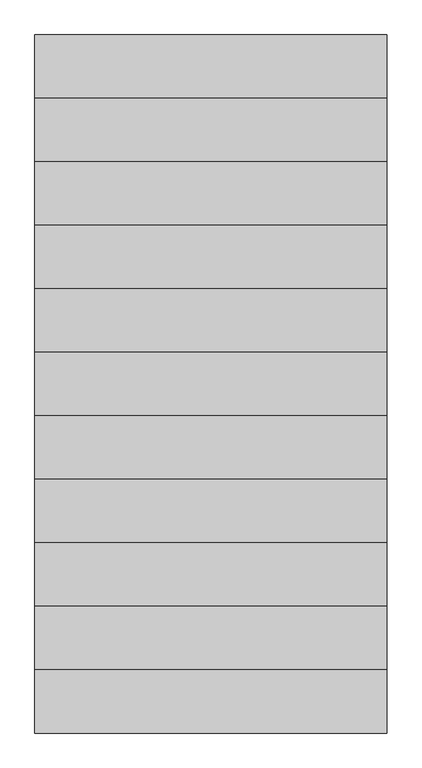
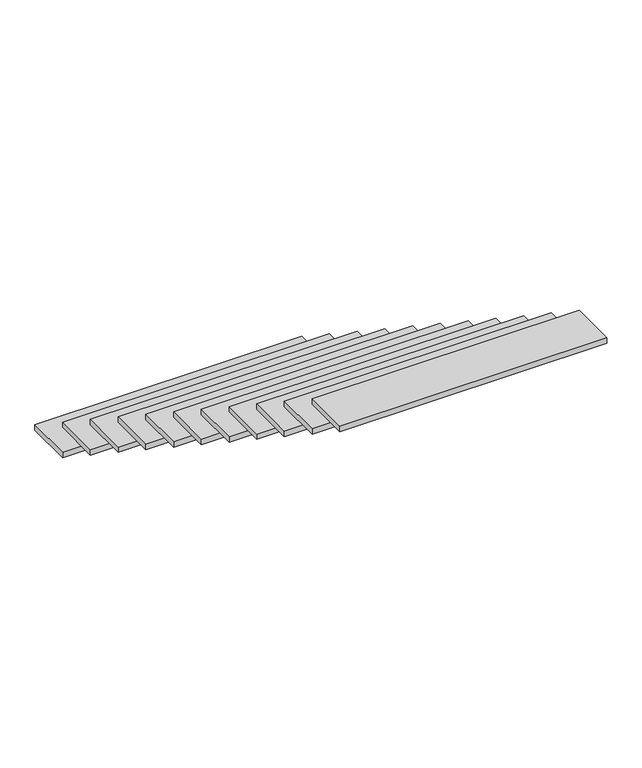
"""IFC4 building model written with IfcOpenShell, lengths in millimetres: stair flight geometry."""

from ifc_helpers import new_model, si_unit, frame, origin, place, context, project, spatial, polyline, outline, extrude, source, transform, mapped, element, save


def stair_flight_fe710d0a(model_context):
    return source(origin(), model_context, "Body", "SweptSolid", [
        extrude(outline(polyline([(16085.3403387, 4647.6066446), (14585.3403387, 4647.6066446), (14585.3403387, 4917.6066446), (16085.3403387, 4917.6066446), (16085.3403387, 4647.6066446)])), frame((0.0, 0.0, 6058.1098901), z_axis=(0.0, 0.0, 1.0), x_axis=(1.0, 0.0, 0.0)), (0.0, 0.0, 1.0), 32.0),
        extrude(outline(polyline([(16085.3403387, 4377.6066446), (14585.3403387, 4377.6066446), (14585.3403387, 4647.6066446), (16085.3403387, 4647.6066446), (16085.3403387, 4377.6066446)])), frame((0.0, 0.0, 6237.2307692), z_axis=(0.0, 0.0, 1.0), x_axis=(1.0, 0.0, 0.0)), (0.0, 0.0, 1.0), 32.0),
        extrude(outline(polyline([(16085.3403387, 4107.6066446), (14585.3403387, 4107.6066446), (14585.3403387, 4377.6066446), (16085.3403387, 4377.6066446), (16085.3403387, 4107.6066446)])), frame((0.0, 0.0, 6416.3516484), z_axis=(0.0, 0.0, 1.0), x_axis=(1.0, 0.0, 0.0)), (0.0, 0.0, 1.0), 32.0),
        extrude(outline(polyline([(16085.3403387, 3837.6066446), (14585.3403387, 3837.6066446), (14585.3403387, 4107.6066446), (16085.3403387, 4107.6066446), (16085.3403387, 3837.6066446)])), frame((0.0, 0.0, 6595.4725275), z_axis=(0.0, 0.0, 1.0), x_axis=(1.0, 0.0, 0.0)), (0.0, 0.0, 1.0), 32.0),
        extrude(outline(polyline([(16085.3403387, 3567.6066446), (14585.3403387, 3567.6066446), (14585.3403387, 3837.6066446), (16085.3403387, 3837.6066446), (16085.3403387, 3567.6066446)])), frame((0.0, 0.0, 6774.5934066), z_axis=(0.0, 0.0, 1.0), x_axis=(1.0, 0.0, 0.0)), (0.0, 0.0, 1.0), 32.0),
        extrude(outline(polyline([(16085.3403387, 3297.6066446), (14585.3403387, 3297.6066446), (14585.3403387, 3567.6066446), (16085.3403387, 3567.6066446), (16085.3403387, 3297.6066446)])), frame((0.0, 0.0, 6953.7142857), z_axis=(0.0, 0.0, 1.0), x_axis=(1.0, 0.0, 0.0)), (0.0, 0.0, 1.0), 32.0),
        extrude(outline(polyline([(16085.3403387, 3027.6066446), (14585.3403387, 3027.6066446), (14585.3403387, 3297.6066446), (16085.3403387, 3297.6066446), (16085.3403387, 3027.6066446)])), frame((0.0, 0.0, 7132.8351648), z_axis=(0.0, 0.0, 1.0), x_axis=(1.0, 0.0, 0.0)), (0.0, 0.0, 1.0), 32.0),
        extrude(outline(polyline([(16085.3403387, 2757.6066446), (14585.3403387, 2757.6066446), (14585.3403387, 3027.6066446), (16085.3403387, 3027.6066446), (16085.3403387, 2757.6066446)])), frame((0.0, 0.0, 7311.956044), z_axis=(0.0, 0.0, 1.0), x_axis=(1.0, 0.0, 0.0)), (0.0, 0.0, 1.0), 32.0),
        extrude(outline(polyline([(16085.3403387, 2487.6066446), (14585.3403387, 2487.6066446), (14585.3403387, 2757.6066446), (16085.3403387, 2757.6066446), (16085.3403387, 2487.6066446)])), frame((0.0, 0.0, 7491.0769231), z_axis=(0.0, 0.0, 1.0), x_axis=(1.0, 0.0, 0.0)), (0.0, 0.0, 1.0), 32.0),
        extrude(outline(polyline([(16085.3403387, 2217.6066446), (14585.3403387, 2217.6066446), (14585.3403387, 2487.6066446), (16085.3403387, 2487.6066446), (16085.3403387, 2217.6066446)])), frame((0.0, 0.0, 7670.1978022), z_axis=(0.0, 0.0, 1.0), x_axis=(1.0, 0.0, 0.0)), (0.0, 0.0, 1.0), 32.0),
        extrude(outline(polyline([(16085.3403387, 1947.6066446), (14585.3403387, 1947.6066446), (14585.3403387, 2217.6066446), (16085.3403387, 2217.6066446), (16085.3403387, 1947.6066446)])), frame((0.0, 0.0, 7849.3186813), z_axis=(0.0, 0.0, 1.0), x_axis=(1.0, 0.0, 0.0)), (0.0, 0.0, 1.0), 32.0),
    ])


if __name__ == "__main__":
    model = new_model("IFC4")
    model_context = context("Model", 3, world=origin())
    ifc_project = project(units=[si_unit("LENGTHUNIT", "METRE", prefix="MILLI")], contexts=[model_context])
    site = spatial("IfcSite", under=ifc_project)
    building = spatial("IfcBuilding", under=site)
    placement = place(None, origin())
    stair_flight_shape = stair_flight_fe710d0a(model_context)
    element("IfcStairFlight", 1, at=placement, inside=building, context=model_context, shape_type="MappedRepresentation", body=[
        mapped(stair_flight_shape, transform((0.0, 0.0, 0.0), x_axis=(1.0, 0.0, 0.0), y_axis=(0.0, 1.0, 0.0), z_axis=(0.0, 0.0, 1.0))),
    ])
    save(model, "model.ifc")

# Revit data of these elements
# Element 1 (IfcStairFlight)
#   Materials on its faces: "철강"
# Materials
#   "철강": class "Generic", colour RGB 143 142 141, transparency 0, Description = "철골+가공조립+세우기", Cost = 0
